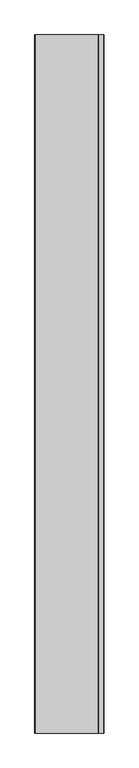
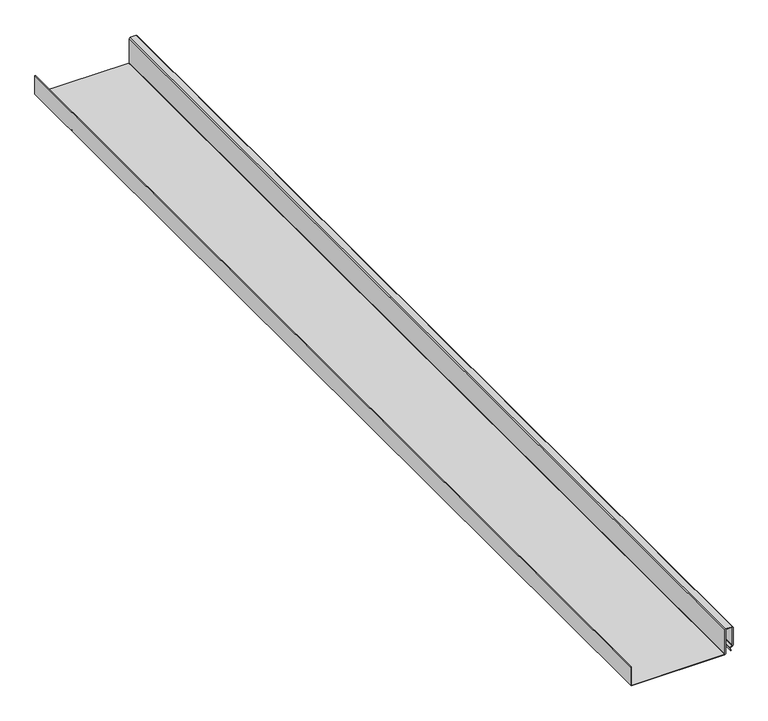
"""IFC4 building model written with IfcOpenShell, lengths in millimetres: proxy geometry, BEND PANEL006 6507 : BEND PANEL006 6507."""

from ifc_helpers import new_model, si_unit, frame, origin, place, context, project, spatial, polyline, outline, extrude, source, transform, mapped, element, save


def generic_models_980f5cdc(model_context):
    return source(origin(), model_context, "Body", "SweptSolid", [
        extrude(outline(polyline([(44154.6016709, 5566.2044341), (44159.2233864, 5564.0492928), (44160.1545891, 5564.3882229), (44162.0840579, 5568.5259314), (44163.9343079, 5569.6973823), (44200.1942886, 5569.6973823), (44202.2899085, 5567.6017624), (44202.2899085, 5555.917225), (44200.1942886, 5553.8216051), (44151.2171561, 5553.8216051), (44150.5164401, 5553.1208891), (44150.5164401, 5372.9642652), (44151.2184658, 5372.2622396), (44187.9858128, 5372.2622396), (44187.9858128, 5371.0716146), (44150.7252927, 5371.0716146), (44149.3258151, 5372.4710922), (44149.3258151, 5553.6140621), (44150.7239831, 5555.0122301), (44199.7011155, 5555.0122301), (44201.0992835, 5556.410398), (44201.0992835, 5567.1085894), (44199.7011156, 5568.5067573), (44164.2795313, 5568.5067573), (44163.015698, 5567.7065851), (44161.0252349, 5563.4380754), (44159.1671731, 5562.7617962), (44154.0984911, 5565.1253614), (44154.6016709, 5566.2044341)])), frame((0.0, -1052.8906574, 0.0), z_axis=(0.0, 1.0, 0.0), x_axis=(0.0, 0.0, 1.0)), (0.0, 0.0, 1.0), 1999.85),
    ])


if __name__ == "__main__":
    model = new_model("IFC4")
    model_context = context("Model", 3, world=origin())
    ifc_project = project(units=[si_unit("LENGTHUNIT", "METRE", prefix="MILLI")], contexts=[model_context])
    site = spatial("IfcSite", under=ifc_project)
    building = spatial("IfcBuilding", under=site)
    placement = place(None, origin())
    generic_models_shape = generic_models_980f5cdc(model_context)
    element("IfcBuildingElementProxy", 1, Name="BEND PANEL006 6507 : BEND PANEL006 6507", ObjectType="BEND PANEL006 6507 : BEND PANEL006 6507", at=placement, inside=building, context=model_context, shape_type="MappedRepresentation", body=[
        mapped(generic_models_shape, transform((0.0, 0.0, 0.0), x_axis=(1.0, 0.0, 0.0), y_axis=(0.0, 1.0, 0.0), z_axis=(0.0, 0.0, 1.0))),
    ])
    save(model, "model.ifc")

# Revit data of these elements
# Type "BEND PANEL006 6507 : BEND PANEL006 6507"
#   NameOverride = "BEND PANEL006"
# Element 1 (IfcBuildingElementProxy, "BEND PANEL006 6507 : BEND PANEL006 6507")
#   Materials on its faces: "STANDING SEAM METAL ROOF FOLLOW MANU. RECOMMENDED EDGE/TRANSITION DETAILS"
# Materials
#   "STANDING SEAM METAL ROOF FOLLOW MANU. RECOMMENDED EDGE/TRANSITION DETAILS": class "Unassigned", colour RGB 128 128 128, transparency 0
